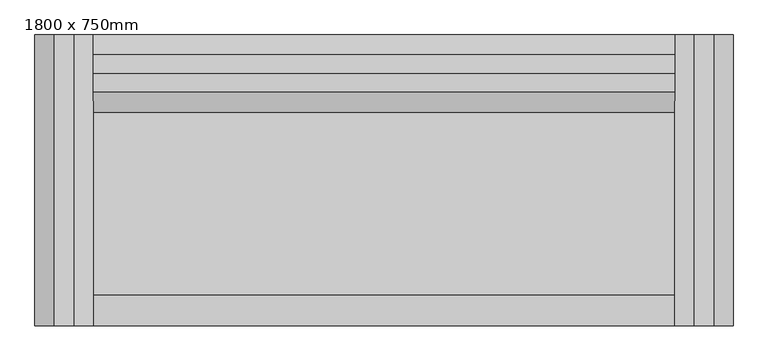
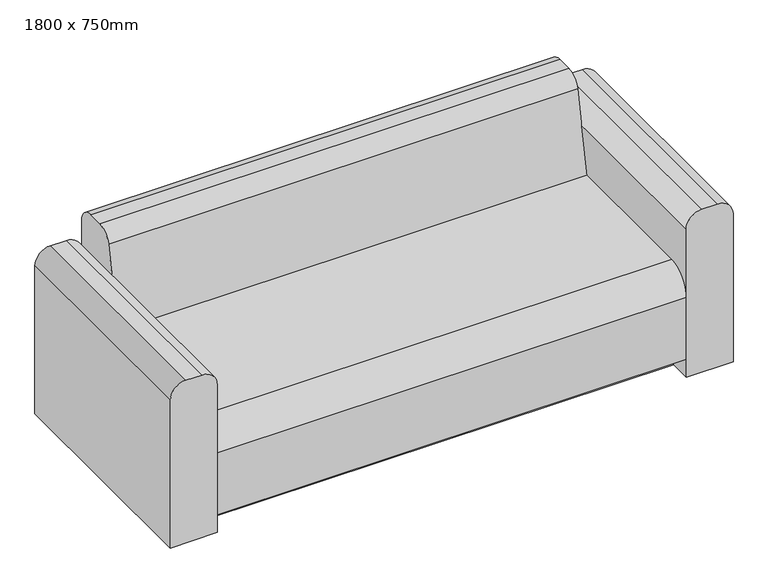
"""IFC4 building model written with IfcOpenShell, lengths in millimetres: furniture geometry, ソファ－I型 : 1800 x 750mm."""

import ifcopenshell
import ifcopenshell.guid

model = None  # the IFC model being written
_history = None  # IfcOwnerHistory: only IFC2X3 demands one
_inside = {}  # id of a spatial element -> (the spatial element, [elements in it])
_under = {}  # id of a project, library or spatial element -> (it, [spatial elements below it])
_declared = {}  # id of a project -> (the project, [libraries it declares])
_typed = {}  # id of a type object -> (the type object, [elements of that type])
_made_of = {}  # id of a material, layer set ... -> (it, [elements and type objects made of it])


def new_model(schema):
    """Start an empty IFC model of exactly this schema.

    Asked for "IFC4X3", IfcOpenShell would pick the latest addendum, in which some entities
    have other attributes; the version numbers below select the first issue.
    IFC2X3 requires an IfcOwnerHistory on every rooted entity: one is made here for all.
    """
    global model, _history
    if schema == "IFC4X3":
        model = ifcopenshell.file(schema_version=(4, 3, 0, 0))
    else:
        model = ifcopenshell.file(schema=schema)
    _inside.clear()
    _under.clear()
    _declared.clear()
    _typed.clear()
    _made_of.clear()
    _history = None
    if model.schema == "IFC2X3":
        org = make("IfcOrganization", Name="unknown")
        user = make(
            "IfcPersonAndOrganization",
            ThePerson=make("IfcPerson", FamilyName="unknown"),
            TheOrganization=org,
        )
        app = make(
            "IfcApplication",
            ApplicationDeveloper=org,
            Version="unknown",
            ApplicationFullName="unknown",
            ApplicationIdentifier="unknown",
        )
        _history = make(
            "IfcOwnerHistory",
            OwningUser=user,
            OwningApplication=app,
            ChangeAction="ADDED",
            CreationDate=0,
        )
    return model


def make(cls, **values):
    """One entity of the class cls with the attributes given. An attribute that is None is left unset."""
    return model.create_entity(
        cls, **{name: value for name, value in values.items() if value is not None}
    )


def rooted(cls, **values):
    """An entity with a GlobalId (a new one), such as an element, a storey or a relation."""
    return make(cls, GlobalId=ifcopenshell.guid.new(), OwnerHistory=_history, **values)


def si_unit(unit_type, name, prefix=None):
    """IfcSIUnit, for example si_unit("LENGTHUNIT", "METRE", prefix="MILLI")."""
    return make("IfcSIUnit", UnitType=unit_type, Prefix=prefix, Name=name)


def assignment(units):
    """IfcUnitAssignment: the units of a project."""
    return None if units is None else make("IfcUnitAssignment", Units=units)


def point(xyz):
    """IfcCartesianPoint."""
    return None if xyz is None else make("IfcCartesianPoint", Coordinates=xyz)


def direction(xyz):
    """IfcDirection."""
    return None if xyz is None else make("IfcDirection", DirectionRatios=xyz)


def frame(location, z_axis=None, x_axis=None):
    """IfcAxis2Placement3D, a coordinate frame: its origin and axes. An axis left out is left unset."""
    return make(
        "IfcAxis2Placement3D",
        Location=point(location),
        Axis=direction(z_axis),
        RefDirection=direction(x_axis),
    )


def frame_2d(location, x_axis=None):
    """IfcAxis2Placement2D, a coordinate frame in the plane: its origin and x axis."""
    return make(
        "IfcAxis2Placement2D", Location=point(location), RefDirection=direction(x_axis)
    )


def origin():
    """The frame at (0, 0, 0) with its axes left unset."""
    return frame((0.0, 0.0, 0.0))


def place(relative_to, where):
    """IfcLocalPlacement: puts the frame where relative to a parent placement (None: the world)."""
    return make(
        "IfcLocalPlacement", PlacementRelTo=relative_to, RelativePlacement=where
    )


def context(
    kind, dimensions, precision=None, world=None, true_north=None, identifier=None
):
    """IfcGeometricRepresentationContext, for example the 3D "Model" context."""
    return make(
        "IfcGeometricRepresentationContext",
        ContextIdentifier=identifier,
        ContextType=kind,
        CoordinateSpaceDimension=dimensions,
        Precision=precision,
        WorldCoordinateSystem=world,
        TrueNorth=true_north,
    )


def project(units=None, contexts=None):
    """IfcProject with its units and contexts."""
    return rooted(
        "IfcProject",
        Name="project",
        RepresentationContexts=contexts,
        UnitsInContext=assignment(units),
    )


def spatial(cls, under=None, at=None, **own):
    """A site, building, storey or space (cls), placed at a placement, below another one or the project."""
    s = rooted(cls, ObjectPlacement=at, **own)
    if under is not None:
        _under.setdefault(under.id(), (under, []))[1].append(s)
    return s


def polyline(points):
    """IfcPolyline through the points."""
    return make("IfcPolyline", Points=[point(p) for p in points])


def circle_curve(where, radius):
    """IfcCircle in the frame where."""
    return make("IfcCircle", Position=where, Radius=radius)


def trimmed(basis, trim1, trim2, sense, master):
    """IfcTrimmedCurve: the piece of a basis curve between two trims."""
    return make(
        "IfcTrimmedCurve",
        BasisCurve=basis,
        Trim1=trim1,
        Trim2=trim2,
        SenseAgreement=sense,
        MasterRepresentation=master,
    )


def segment(curve, same_sense, transition):
    """IfcCompositeCurveSegment."""
    return make(
        "IfcCompositeCurveSegment",
        Transition=transition,
        SameSense=same_sense,
        ParentCurve=curve,
    )


def composite_curve(segments, self_intersect=None):
    """IfcCompositeCurve: segments joined end to end."""
    return make("IfcCompositeCurve", Segments=segments, SelfIntersect=self_intersect)


def outline(outer, holes=None, kind="AREA"):
    """IfcArbitraryClosedProfileDef: a profile drawn as a closed curve; with holes, ...WithVoids."""
    if holes is None:
        return make("IfcArbitraryClosedProfileDef", ProfileType=kind, OuterCurve=outer)
    return make(
        "IfcArbitraryProfileDefWithVoids",
        ProfileType=kind,
        OuterCurve=outer,
        InnerCurves=holes,
    )


def extrude(swept, where, along, depth):
    """IfcExtrudedAreaSolid: the profile swept, set in the frame where, extruded along a direction by depth."""
    return make(
        "IfcExtrudedAreaSolid",
        SweptArea=swept,
        Position=where,
        ExtrudedDirection=direction(along),
        Depth=depth,
    )


def shape(context_of_items, identifier, shape_type, items):
    """IfcShapeRepresentation: the items that make up one representation, for example the "Body"."""
    return make(
        "IfcShapeRepresentation",
        ContextOfItems=context_of_items,
        RepresentationIdentifier=identifier,
        RepresentationType=shape_type,
        Items=items,
    )


def source(mapping_origin, context_of_items, identifier, shape_type, items):
    """IfcRepresentationMap: a shape defined once, which mapped items show again and again."""
    return make(
        "IfcRepresentationMap",
        MappingOrigin=mapping_origin,
        MappedRepresentation=shape(context_of_items, identifier, shape_type, items),
    )


def transform(
    local_origin,
    x_axis=None,
    y_axis=None,
    z_axis=None,
    scale=None,
    scale2=None,
    scale3=None,
    uniform=True,
):
    """IfcCartesianTransformationOperator3D, or its non-uniform kind. x_axis, y_axis, z_axis: its Axis1, 2, 3."""
    if uniform:
        return make(
            "IfcCartesianTransformationOperator3D",
            Axis1=direction(x_axis),
            Axis2=direction(y_axis),
            LocalOrigin=point(local_origin),
            Scale=scale,
            Axis3=direction(z_axis),
        )
    return make(
        "IfcCartesianTransformationOperator3DnonUniform",
        Axis1=direction(x_axis),
        Axis2=direction(y_axis),
        LocalOrigin=point(local_origin),
        Scale=scale,
        Axis3=direction(z_axis),
        Scale2=scale2,
        Scale3=scale3,
    )


def mapped(mapping_source, mapping_target):
    """IfcMappedItem: shows the shape of a source again, moved by a transform."""
    return make(
        "IfcMappedItem", MappingSource=mapping_source, MappingTarget=mapping_target
    )


def made_of(thing, what):
    """Note that an element or type object is made of a material, layer set ...; save() writes the relation."""
    if what is not None:
        _made_of.setdefault(what.id(), (what, []))[1].append(thing)
    return thing


def element(
    cls,
    number,
    at=None,
    inside=None,
    cuts=None,
    type_object=None,
    material=None,
    context=None,
    identifier="Body",
    shape_type=None,
    held_by="IfcProductDefinitionShape",
    body=None,
    shapes=None,
    **own,
):
    """One element of the class cls, such as IfcWall. Its Tag is "e" and its number.

    at: its placement. inside: the storey or other place that contains it. cuts: it is an
    opening in that element (IfcRelVoidsElement). A single representation is given by context,
    identifier, shape_type and body (its items); several are given by shapes. held_by: the class
    of the entity that holds the representations. save() writes the other relations.
    """
    e = rooted(cls, Tag="e%d" % number, ObjectPlacement=at, **own)
    if body is not None:
        shapes = [shape(context, identifier, shape_type, body)]
    if shapes is not None:
        e.Representation = make(held_by, Representations=shapes)
    if inside is not None:
        _inside.setdefault(inside.id(), (inside, []))[1].append(e)
    if cuts is not None:
        rooted(
            "IfcRelVoidsElement", RelatingBuildingElement=cuts, RelatedOpeningElement=e
        )
    if type_object is not None:
        _typed.setdefault(type_object.id(), (type_object, []))[1].append(e)
    return made_of(e, material)


def aggregate(whole, parts):
    """IfcRelAggregates: a whole, such as a stair, and the parts it consists of."""
    return rooted("IfcRelAggregates", RelatingObject=whole, RelatedObjects=parts)


def save(model, path):
    """Write the relations noted so far, then the file.

    IfcRelAggregates (storeys below a building ...), IfcRelContainedInSpatialStructure (elements
    in a storey), IfcRelDefinesByType, IfcRelAssociatesMaterial and IfcRelDeclares: one each for
    every whole, place, type object, material and project.
    """
    for whole, parts in _under.values():
        aggregate(whole, parts)
    for where, things in _inside.values():
        rooted(
            "IfcRelContainedInSpatialStructure",
            RelatedElements=things,
            RelatingStructure=where,
        )
    for kind, things in _typed.values():
        rooted("IfcRelDefinesByType", RelatedObjects=things, RelatingType=kind)
    for what, things in _made_of.values():
        rooted("IfcRelAssociatesMaterial", RelatedObjects=things, RelatingMaterial=what)
    for by, libraries in _declared.values():
        rooted("IfcRelDeclares", RelatingContext=by, RelatedDefinitions=libraries)
    model.write(path)


def furniture_1800_x_750mm_b4778df9(model_context):
    return source(origin(), model_context, "Body", "SweptSolid", [
        extrude(outline(composite_curve([segment(trimmed(circle_curve(frame_2d((500.0, -850.0)), 50.0), [point((550.0, -850.0))], [point((500.0, -900.0))], False, "CARTESIAN"), True, "CONTINUOUS"), segment(polyline([(500.0, -900.0), (0.0, -900.0), (0.0, -750.0), (500.0, -750.0)]), True, "CONTINUOUS"), segment(trimmed(circle_curve(frame_2d((500.0, -800.0)), 50.0), [point((500.0, -750.0))], [point((550.0, -800.0))], False, "CARTESIAN"), True, "CONTINUOUS"), segment(polyline([(550.0, -800.0), (550.0, -850.0)]), True, "CONTINUOUS")], self_intersect=False)), frame((0.0, -375.0, 0.0), z_axis=(0.0, 1.0, 0.0), x_axis=(0.0, 0.0, 1.0)), (0.0, 0.0, 1.0), 750.0),
        extrude(outline(composite_curve([segment(polyline([(550.0, 850.0), (550.0, 800.0)]), True, "CONTINUOUS"), segment(trimmed(circle_curve(frame_2d((500.0, 800.0)), 50.0), [point((550.0, 800.0))], [point((500.0, 750.0))], False, "CARTESIAN"), True, "CONTINUOUS"), segment(polyline([(500.0, 750.0), (0.0, 750.0), (0.0, 900.0), (500.0, 900.0)]), True, "CONTINUOUS"), segment(trimmed(circle_curve(frame_2d((500.0, 850.0)), 50.0), [point((500.0, 900.0))], [point((550.0, 850.0))], False, "CARTESIAN"), True, "CONTINUOUS")], self_intersect=False)), frame((0.0, -375.0, 0.0), z_axis=(0.0, 1.0, 0.0), x_axis=(0.0, 0.0, 1.0)), (0.0, 0.0, 1.0), 750.0),
        extrude(outline(composite_curve([segment(trimmed(circle_curve(frame_2d((275.9901951, 600.0)), 50.0), [point((226.9611614, 609.8058068))], [point((275.9901951, 650.0))], False, "CARTESIAN"), True, "CONTINUOUS"), segment(polyline([(275.9901951, 650.0), (325.0, 650.0)]), True, "CONTINUOUS"), segment(trimmed(circle_curve(frame_2d((325.0, 600.0)), 50.0), [point((325.0, 650.0))], [point((375.0, 600.0))], False, "CARTESIAN"), True, "CONTINUOUS"), segment(polyline([(375.0, 600.0), (375.0, 0.0), (-305.0, 0.0), (-305.0, 60.0), (-375.0, 60.0), (-375.0, 270.0)]), True, "CONTINUOUS"), segment(trimmed(circle_curve(frame_2d((-295.0, 270.0)), 80.0), [point((-375.0, 270.0))], [point((-295.0, 350.0))], False, "CARTESIAN"), True, "CONTINUOUS"), segment(polyline([(-295.0, 350.0), (175.0, 350.0), (226.9611614, 609.8058068)]), True, "CONTINUOUS")], self_intersect=False)), frame((-750.0, 0.0, 0.0), z_axis=(1.0, 0.0, 0.0), x_axis=(0.0, 1.0, 0.0)), (0.0, 0.0, 1.0), 1500.0),
    ])


if __name__ == "__main__":
    model = new_model("IFC4")
    model_context = context("Model", 3, world=origin())
    ifc_project = project(units=[si_unit("LENGTHUNIT", "METRE", prefix="MILLI")], contexts=[model_context])
    site = spatial("IfcSite", under=ifc_project)
    building = spatial("IfcBuilding", under=site)
    placement = place(None, origin())
    furniture_1800_x_750mm_shape = furniture_1800_x_750mm_b4778df9(model_context)
    element("IfcFurniture", 1, ObjectType="ソファ－I型 : 1800 x 750mm", at=placement, inside=building, context=model_context, shape_type="MappedRepresentation", body=[
        mapped(furniture_1800_x_750mm_shape, transform((0.0, 0.0, 0.0), x_axis=(1.0, 0.0, 0.0), y_axis=(0.0, 1.0, 0.0), z_axis=(0.0, 0.0, 1.0))),
    ])
    save(model, "model.ifc")

# Revit data of these elements
# Project information
#   プロジェクト発行日 = "発行日"
#   プロジェクト ステータス = "プロジェクト ステータス"
#   クライアント名 = "オーナ"
#   計画地住所 = "ここにアドレスを入力"
#   プロジェクト名 = "プロジェクト名"
#   プロジェクト番号 = "0001"
# Type "ソファ－I型 : 1800 x 750mm"
#   Keynote = "12490.Y1"
#   座面高さ = 350 mm
#   幅 = 1800 mm
#   奥行き = 750 mm
#   本体 = モチアミ - 無地 - グレー
#   Default Elevation = 0
# Element 1 (IfcFurniture, "ソファ－I型 : 1800 x 750mm")
#   Materials on its faces: "モチアミ - 無地 - グレー"
# Materials
#   "モチアミ - 無地 - グレー": class "モチアミ", colour RGB 65 63 65, transparency 0, Cost = 0
